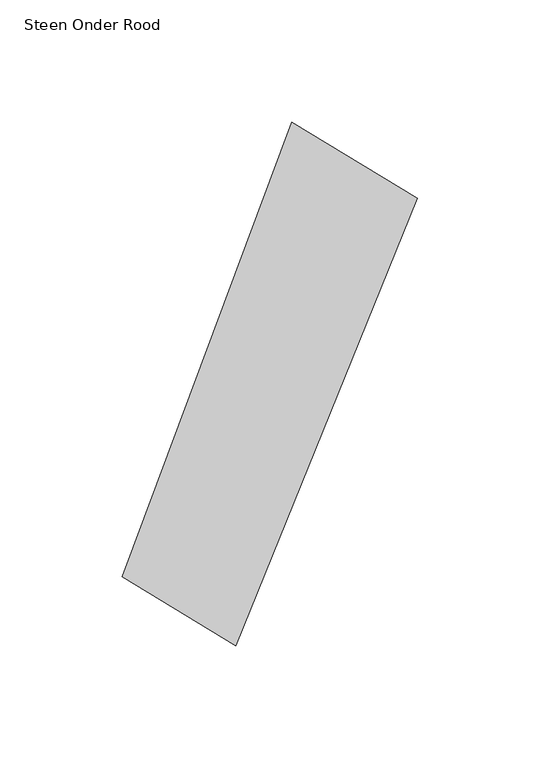
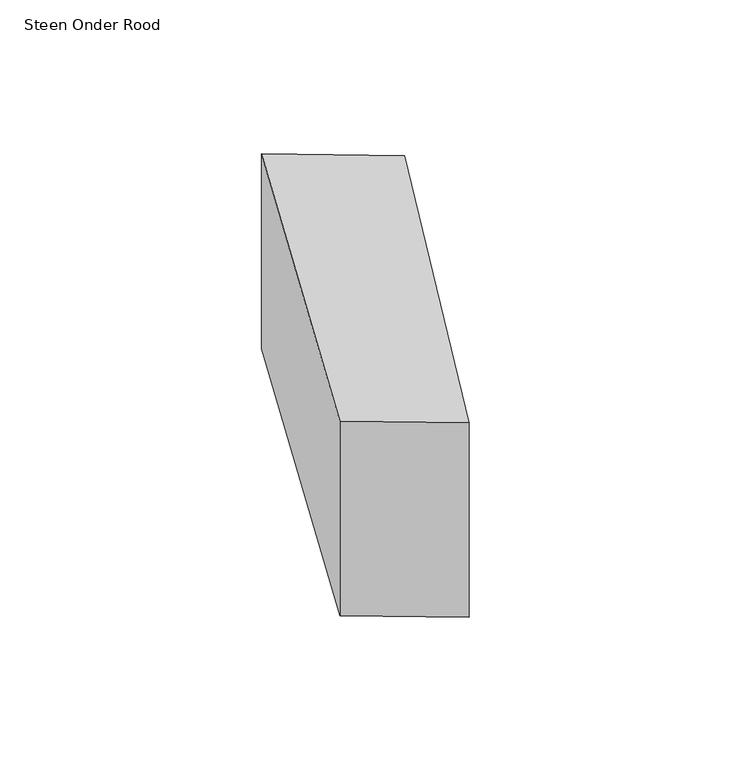
"""IFC4 building model written with IfcOpenShell, lengths in millimetres: proxy geometry, 00_GMA_steen_versie_4 : Steen Onder Rood."""

from ifc_helpers import new_model, si_unit, origin, origin_with_axes, place, context, project, spatial, polyline, outline, extrude, source, transform, mapped, element, save


def steen_onder_rood_96d146e5(model_context):
    return source(origin(), model_context, "Body", "SweptSolid", [
        extrude(outline(polyline([(137.5024385, 160.4006196), (63.1729684, -22.6540172), (16.7362284, 5.5054327), (86.1971343, 191.5369363), (137.5024385, 160.4006196)])), origin_with_axes(), (0.0, 0.0, 1.0), 100.0),
    ])


if __name__ == "__main__":
    model = new_model("IFC4")
    model_context = context("Model", 3, world=origin())
    ifc_project = project(units=[si_unit("LENGTHUNIT", "METRE", prefix="MILLI")], contexts=[model_context])
    site = spatial("IfcSite", under=ifc_project)
    building = spatial("IfcBuilding", under=site)
    placement = place(None, origin())
    steen_onder_rood_shape = steen_onder_rood_96d146e5(model_context)
    element("IfcBuildingElementProxy", 1, Name="00_GMA_steen_versie_4 : Steen Onder Rood", ObjectType="00_GMA_steen_versie_4 : Steen Onder Rood", at=placement, inside=building, context=model_context, shape_type="MappedRepresentation", body=[
        mapped(steen_onder_rood_shape, transform((0.0, 0.0, 0.0), x_axis=(1.0, 0.0, 0.0), y_axis=(0.0, 1.0, 0.0), z_axis=(0.0, 0.0, 1.0))),
    ])
    save(model, "model.ifc")

# Revit data of these elements
# Type "00_GMA_steen_versie_4 : Steen Onder Rood"
#   StootVoegHalfBoven [instance default] = 5 mm
#   StootVoegHalf [instance default] = 5 mm
#   StootVoegBreedteOnder = 10 mm
#   StootVoegBreedteBoven = 10 mm
#   Steendikte = 100 mm
#   LintVoegOnderHalf = 0 mm
#   LintVoegOnder = 0 mm
#   LintVoegBovenHalf = 5 mm
#   LintVoegBoven = 10 mm
#   materiaal = 21_steen_rood
#   MateriaalVoeg = none
#   Default Elevation = 0
# Element 1 (IfcBuildingElementProxy, "00_GMA_steen_versie_4 : Steen Onder Rood")
#   Materials on its faces: "21_steen_rood"
# Materials
#   "21_steen_rood": class "Unassigned", colour RGB 213 111 43, transparency 0, Cost = 0
